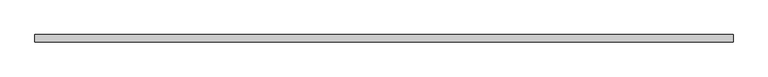
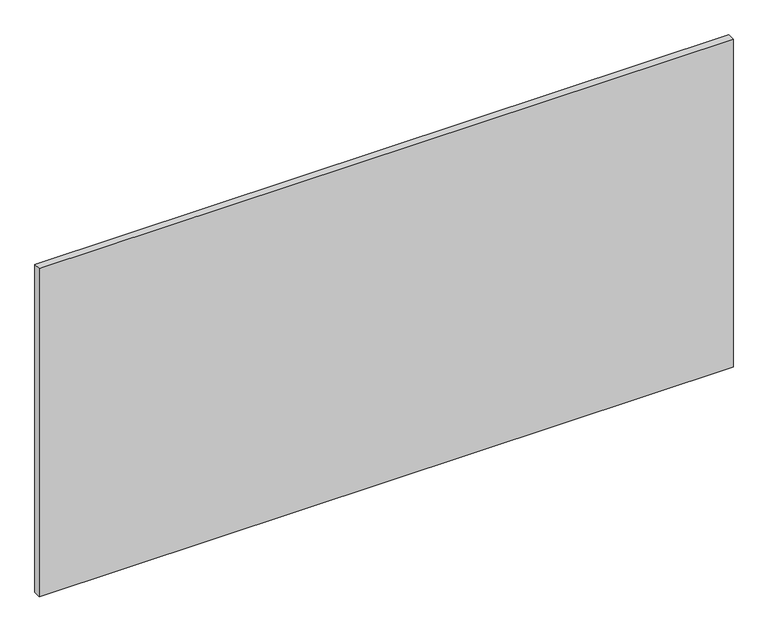
"""IFC4 building model written with IfcOpenShell, lengths in millimetres: proxy geometry, Vertical furring:Vertical furring:3:Vertical furring:3 : Vertical furring:Vertical furring:300288:353074:Vertical furring:3:Vertical furring:3 : Vertical furring:Vertical furring:300288:353074 : Vertical furring:Vertical furring:3:Vertical furring:3 : Vertical furring:Vertical furring:300288:353074:1 : Vertical furring:Vertical furring:3:Vertical furring:3 : Vertical furring:Vertical furring:300288:353074:Vertical furring:3:Vertical furring:3 : Vertical furring:Vertical furring:300288:353074 : Vertical furring:Vertical furring:3:Vertical furring:3 : Vertical furring:Vertical furring:300288:353074:301917."""

from ifc_helpers import new_model, si_unit, frame, origin, place, context, project, spatial, polyline, outline, extrude, source, transform, mapped, element, save


def generic_models_33611fa6(model_context):
    return source(origin(), model_context, "Body", "SweptSolid", [
        extrude(outline(polyline([(570452.6367239, -579022.9163841), (572891.0367239, -579022.9163841), (572891.0367239, -579048.3163841), (570452.6367239, -579048.3163841), (570452.6367239, -579022.9163841)])), frame((0.0, 0.0, 2438.4), z_axis=(0.0, 0.0, 1.0), x_axis=(1.0, 0.0, 0.0)), (0.0, 0.0, 1.0), 1219.2),
    ])


if __name__ == "__main__":
    model = new_model("IFC4")
    model_context = context("Model", 3, world=origin())
    ifc_project = project(units=[si_unit("LENGTHUNIT", "METRE", prefix="MILLI")], contexts=[model_context])
    site = spatial("IfcSite", under=ifc_project)
    building = spatial("IfcBuilding", under=site)
    placement = place(None, origin())
    generic_models_shape = generic_models_33611fa6(model_context)
    element("IfcBuildingElementProxy", 1, Name="Vertical furring:Vertical furring:3:Vertical furring:3 : Vertical furring:Vertical furring:300288:353074:Vertical furring:3:Vertical furring:3 : Vertical furring:Vertical furring:300288:353074 : Vertical furring:Vertical furring:3:Vertical furring:3 : Vertical furring:Vertical furring:300288:353074:1 : Vertical furring:Vertical furring:3:Vertical furring:3 : Vertical furring:Vertical furring:300288:353074:Vertical furring:3:Vertical furring:3 : Vertical furring:Vertical furring:300288:353074 : Vertical furring:Vertical furring:3:Vertical furring:3 : Vertical furring:Vertical furring:300288:353074:301917", ObjectType="Vertical furring:Vertical furring:3:Vertical furring:3 : Vertical furring:Vertical furring:300288:353074:Vertical furring:3:Vertical furring:3 : Vertical furring:Vertical furring:300288:353074 : Vertical furring:Vertical furring:3:Vertical furring:3 : Vertical furring:Vertical furring:300288:353074:1 : Vertical furring:Vertical furring:3:Vertical furring:3 : Vertical furring:Vertical furring:300288:353074:Vertical furring:3:Vertical furring:3 : Vertical furring:Vertical furring:300288:353074 : Vertical furring:Vertical furring:3:Vertical furring:3 : Vertical furring:Vertical furring:300288:353074:301917", at=placement, inside=building, context=model_context, shape_type="MappedRepresentation", body=[
        mapped(generic_models_shape, transform((0.0, 0.0, 0.0), x_axis=(1.0, 0.0, 0.0), y_axis=(0.0, 1.0, 0.0), z_axis=(0.0, 0.0, 1.0))),
    ])
    save(model, "model.ifc")

# Revit data of these elements
# Type "Vertical furring:Vertical furring:3:Vertical furring:3 : Vertical furring:Vertical furring:300288:353074:Vertical furring:3:Vertical furring:3 : Vertical furring:Vertical furring:300288:353074 : Vertical furring:Vertical furring:3:Vertical furring:3 : Vertical furring:Vertical furring:300288:353074:1 : Vertical furring:Vertical furring:3:Vertical furring:3 : Vertical furring:Vertical furring:300288:353074:Vertical furring:3:Vertical furring:3 : Vertical furring:Vertical furring:300288:353074 : Vertical furring:Vertical furring:3:Vertical furring:3 : Vertical furring:Vertical furring:300288:353074:301917"
#   NameOverride = "Vertical furring:Vertical furring:3:Vertical furring:3 : Vertical furring:Vertical furring:300288:353074:Vertical furring:3:Vertical furring:3 : Vertical furring:Vertical furring:300288:353074 : Vertical furring:Vertical furring:3:Vertical furring:3 : Vertical furring:Vertical furring:300288:353074:301917"
#   ObjectTypeOverride = "Vertical furring:3:Vertical furring:3 : Vertical furring:Vertical furring:300288:353074 : Vertical furring:Vertical furring:3:Vertical furring:3 : Vertical furring:Vertical furring:300288:353074"
#   Reference = "Vertical furring"
#   Tag = "301917"
# Element 1 (IfcBuildingElementProxy, "Vertical furring:Vertical furring:3:Vertical furring:3 : Vertical furring:Vertical furring:300288:353074:Vertical furring:3:Vertical furring:3 : Vertical furring:Vertical furring:300288:353074 : Vertical furring:Vertical furring:3:Vertical furring:3 : Vertical furring:Vertical furring:300288:353074:1 : Vertical furring:Vertical furring:3:Vertical furring:3 : Vertical furring:Vertical furring:300288:353074:Vertical furring:3:Vertical furring:3 : Vertical furring:Vertical furring:300288:353074 : Vertical furring:Vertical furring:3:Vertical furring:3 : Vertical furring:Vertical furring:300288:353074:301917")
#   Materials on its faces: "1\" MINERAL WOOL BOARD INSULATION - BLACK MAT FACER"
# Materials
#   "1\" MINERAL WOOL BOARD INSULATION - BLACK MAT FACER": class "Unassigned", colour RGB 205 188 106, transparency 0, Cost = 0
